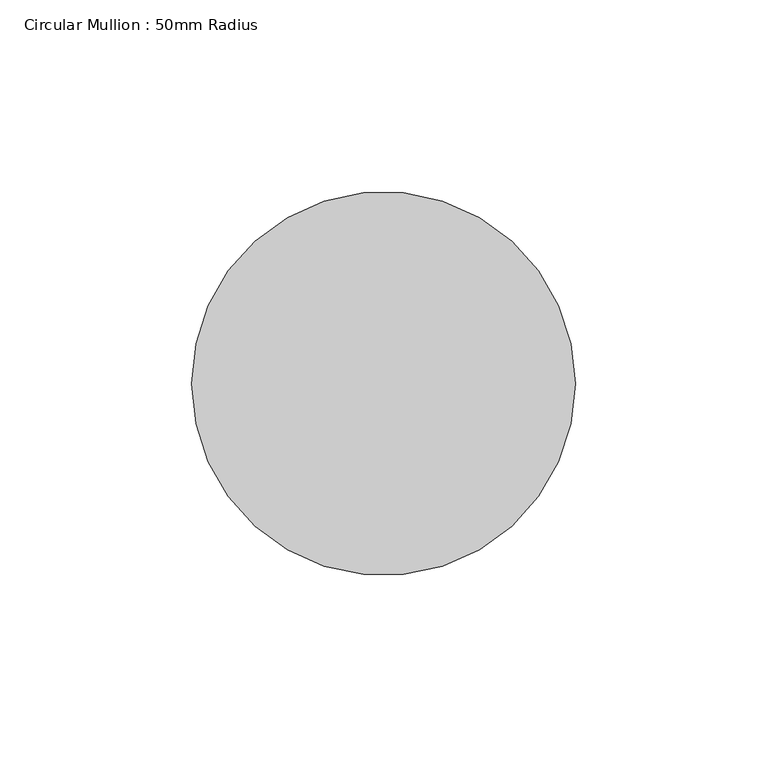
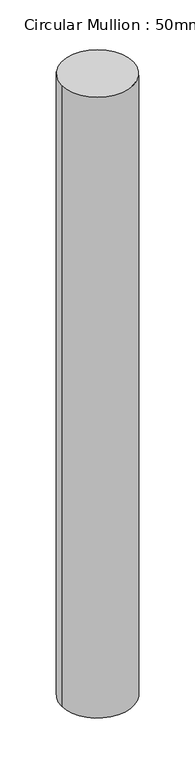
"""IFC4 building model written with IfcOpenShell, lengths in millimetres: member geometry, Circular Mullion : 50mm Radius."""

from ifc_helpers import new_model, si_unit, point, frame, origin, origin_2d, place, context, project, spatial, circle_curve, trimmed, segment, composite_curve, outline, extrude, source, transform, mapped, element, save


def circular_mullion_50mm_radius_9e808e26(model_context):
    return source(origin(), model_context, "Body", "SweptSolid", [
        extrude(outline(composite_curve([segment(trimmed(circle_curve(origin_2d(), 50.0), [point((50.0, 0.0))], [point((-50.0, 0.0))], False, "CARTESIAN"), True, "CONTINUOUS"), segment(trimmed(circle_curve(origin_2d(), 50.0), [point((-50.0, 0.0))], [point((50.0, 0.0))], False, "CARTESIAN"), True, "CONTINUOUS")], self_intersect=False)), frame((0.0, 0.0, -920.0134373), z_axis=(0.0, 0.0, 1.0), x_axis=(1.0, 0.0, 0.0)), (0.0, 0.0, 1.0), 920.0134373),
    ])


if __name__ == "__main__":
    model = new_model("IFC4")
    model_context = context("Model", 3, world=origin())
    ifc_project = project(units=[si_unit("LENGTHUNIT", "METRE", prefix="MILLI")], contexts=[model_context])
    site = spatial("IfcSite", under=ifc_project)
    building = spatial("IfcBuilding", under=site)
    placement = place(None, origin())
    circular_mullion_50mm_radius_shape = circular_mullion_50mm_radius_9e808e26(model_context)
    element("IfcMember", 1, ObjectType="Circular Mullion : 50mm Radius", at=placement, inside=building, context=model_context, shape_type="MappedRepresentation", body=[
        mapped(circular_mullion_50mm_radius_shape, transform((0.0, 0.0, 0.0), x_axis=(1.0, 0.0, 0.0), y_axis=(0.0, 1.0, 0.0), z_axis=(0.0, 0.0, 1.0))),
    ])
    save(model, "model.ifc")

# Revit data of these elements
# Type "Circular Mullion : 50mm Radius"
#   built-in parameter 1007350 = 0.164042 (stored number, unit not read)
# Element 1 (IfcMember, "Circular Mullion : 50mm Radius")
#   Materials on its faces: "Aluminium"
# Materials
#   "Aluminium": class "Metal", colour RGB 247 247 247, transparency 0, Description = "Aluminium 6061", Cost = 0
